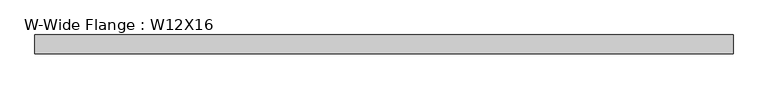
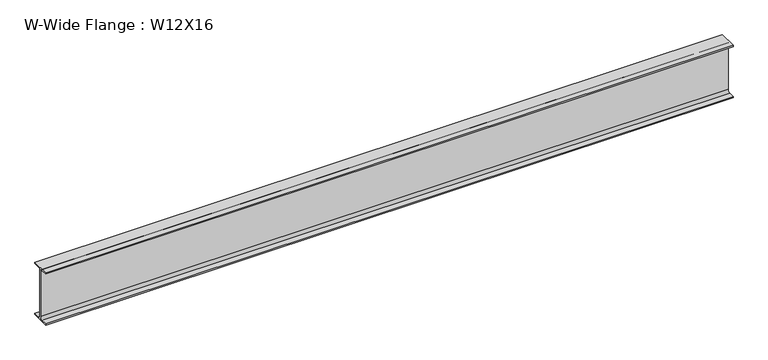
"""IFC4 building model written with IfcOpenShell, lengths in millimetres: beam geometry, W-Wide Flange : W12X16."""

from ifc_helpers import new_model, si_unit, point, frame, frame_2d, origin, place, context, project, spatial, polyline, circle_curve, trimmed, segment, composite_curve, outline, extrude, source, transform, mapped, element, save


def w_wide_flange_w12x16_9e39a167(model_context):
    return source(origin(), model_context, "Body", "SweptSolid", [
        extrude(outline(composite_curve([segment(polyline([(50.673, -145.669), (50.673, -152.4), (-50.673, -152.4), (-50.673, -145.669), (-16.7005, -145.669)]), True, "CONTINUOUS"), segment(trimmed(circle_curve(frame_2d((-16.7005, -131.7625)), 13.9065), [point((-16.7005, -145.669))], [point((-2.794, -131.7625))], True, "CARTESIAN"), True, "CONTINUOUS"), segment(polyline([(-2.794, -131.7625), (-2.794, 131.7625)]), True, "CONTINUOUS"), segment(trimmed(circle_curve(frame_2d((-16.7005, 131.7625)), 13.9065), [point((-2.794, 131.7625))], [point((-16.7005, 145.669))], True, "CARTESIAN"), True, "CONTINUOUS"), segment(polyline([(-16.7005, 145.669), (-50.673, 145.669), (-50.673, 152.4), (50.673, 152.4), (50.673, 145.669), (16.7005, 145.669)]), True, "CONTINUOUS"), segment(trimmed(circle_curve(frame_2d((16.7005, 131.7625)), 13.9065), [point((16.7005, 145.669))], [point((2.794, 131.7625))], True, "CARTESIAN"), True, "CONTINUOUS"), segment(polyline([(2.794, 131.7625), (2.794, -131.7625)]), True, "CONTINUOUS"), segment(trimmed(circle_curve(frame_2d((16.7005, -131.7625)), 13.9065), [point((2.794, -131.7625))], [point((16.7005, -145.669))], True, "CARTESIAN"), True, "CONTINUOUS"), segment(polyline([(16.7005, -145.669), (50.673, -145.669)]), True, "CONTINUOUS")], self_intersect=False)), frame((-1892.3, 0.0, 0.0), z_axis=(1.0, 0.0, 0.0), x_axis=(0.0, 1.0, 0.0)), (0.0, 0.0, 1.0), 3784.6),
    ])


if __name__ == "__main__":
    model = new_model("IFC4")
    model_context = context("Model", 3, world=origin())
    ifc_project = project(units=[si_unit("LENGTHUNIT", "METRE", prefix="MILLI")], contexts=[model_context])
    site = spatial("IfcSite", under=ifc_project)
    building = spatial("IfcBuilding", under=site)
    placement = place(None, origin())
    w_wide_flange_w12x16_shape = w_wide_flange_w12x16_9e39a167(model_context)
    element("IfcBeam", 1, ObjectType="W-Wide Flange : W12X16", at=placement, inside=building, context=model_context, shape_type="MappedRepresentation", body=[
        mapped(w_wide_flange_w12x16_shape, transform((0.0, 0.0, 0.0), x_axis=(1.0, 0.0, 0.0), y_axis=(0.0, 1.0, 0.0), z_axis=(0.0, 0.0, 1.0))),
    ])
    save(model, "model.ifc")

# Revit data of these elements
# Type "W-Wide Flange : W12X16"
#   Assembly Code = "B10"
#   W = 16
#   Length [instance default] = 5' - 0"
#   bf = 0' - 3.99"
#   d = 1' - 0"
#   k = 0' - 0 13/16"
#   k2 = 0' - 0.5475"
#   tf = 0' - 0.265"
#   tw = 0' - 0.22"
#   A = 0.0327083 SF
#   Structural Material [instance default] = Steel ASTM A992
# Element 1 (IfcBeam, "W-Wide Flange : W12X16")
#   Materials on its faces: "Steel ASTM A992"
# Materials
#   "Steel ASTM A992": class "Metal", colour RGB 199 199 199, transparency 0, Description = "Structural steel 50ksi", Cost = 0
